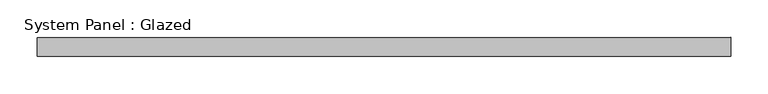
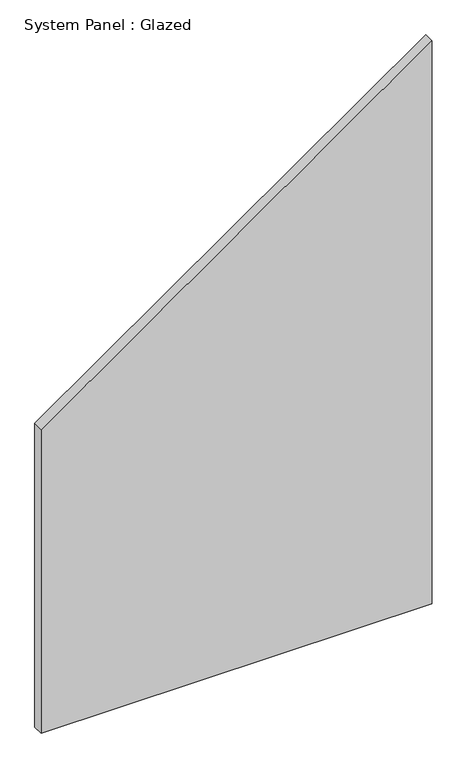
"""IFC4 building model written with IfcOpenShell, lengths in millimetres: plate geometry, System Panel : Glazed."""

from ifc_helpers import new_model, si_unit, frame, origin, place, context, project, spatial, polyline, outline, extrude, source, transform, mapped, element, save


def system_panel_glazed_19015e5b(model_context):
    return source(origin(), model_context, "Body", "SweptSolid", [
        extrude(outline(polyline([(0.0, -462.5), (0.0, 462.5), (1406.7258818, 462.5), (759.0339089, -462.5), (0.0, -462.5)])), frame((0.0, 24.5, 0.0), z_axis=(0.0, 1.0, 0.0), x_axis=(0.0, 0.0, 1.0)), (0.0, 0.0, 1.0), 25.0),
    ])


if __name__ == "__main__":
    model = new_model("IFC4")
    model_context = context("Model", 3, world=origin())
    ifc_project = project(units=[si_unit("LENGTHUNIT", "METRE", prefix="MILLI")], contexts=[model_context])
    site = spatial("IfcSite", under=ifc_project)
    building = spatial("IfcBuilding", under=site)
    placement = place(None, origin())
    system_panel_glazed_shape = system_panel_glazed_19015e5b(model_context)
    element("IfcPlate", 1, ObjectType="System Panel : Glazed", at=placement, inside=building, context=model_context, shape_type="MappedRepresentation", body=[
        mapped(system_panel_glazed_shape, transform((0.0, 0.0, 0.0), x_axis=(1.0, 0.0, 0.0), y_axis=(0.0, 1.0, 0.0), z_axis=(0.0, 0.0, 1.0))),
    ])
    save(model, "model.ifc")

# Revit data of these elements
# Type "System Panel : Glazed"
#   Construction Type Id = "GSP4R"
#   Analytic Construction = "1/8 in Pilkington single glazing"
#   Visual Light Transmittance = 0.9
#   Solar Heat Gain Coefficient = 0.86
#   Heat Transfer Coefficient (U) = 6.7069 W/(m²·K)
#   Define Thermal Properties by = 1
# Element 1 (IfcPlate, "System Panel : Glazed")
#   Materials on its faces: "Glass"
# Materials
#   "Glass": class "Glass", colour RGB 0 128 192, transparency 0.9, Description = "Soda Lime Glass", Cost = 0
